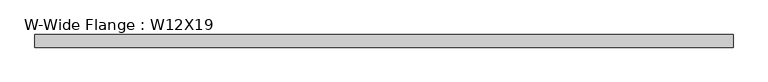
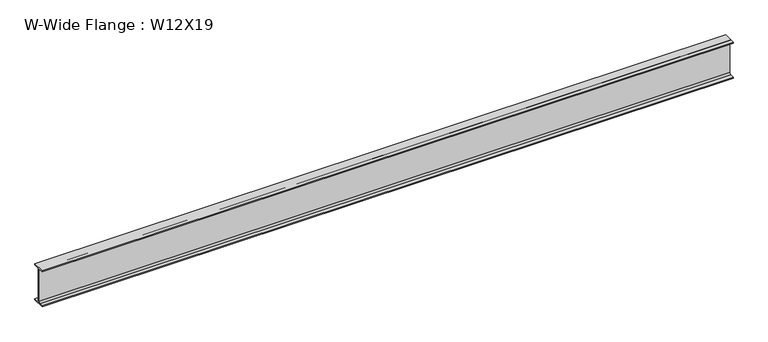
"""IFC4 building model written with IfcOpenShell, lengths in millimetres: beam geometry, W-Wide Flange : W12X19."""

from ifc_helpers import new_model, si_unit, point, frame, frame_2d, origin, place, context, project, spatial, polyline, circle_curve, trimmed, segment, composite_curve, outline, extrude, source, transform, mapped, element, save


def w_wide_flange_w12x19_30f12cce(model_context):
    return source(origin(), model_context, "Body", "SweptSolid", [
        extrude(outline(composite_curve([segment(polyline([(50.927, -146.05), (50.927, -154.94), (-50.927, -154.94), (-50.927, -146.05), (-16.3195, -146.05)]), True, "CONTINUOUS"), segment(trimmed(circle_curve(frame_2d((-16.3195, -132.715)), 13.335), [point((-16.3195, -146.05))], [point((-2.9845, -132.715))], True, "CARTESIAN"), True, "CONTINUOUS"), segment(polyline([(-2.9845, -132.715), (-2.9845, 132.715)]), True, "CONTINUOUS"), segment(trimmed(circle_curve(frame_2d((-16.3195, 132.715)), 13.335), [point((-2.9845, 132.715))], [point((-16.3195, 146.05))], True, "CARTESIAN"), True, "CONTINUOUS"), segment(polyline([(-16.3195, 146.05), (-50.927, 146.05), (-50.927, 154.94), (50.927, 154.94), (50.927, 146.05), (16.3195, 146.05)]), True, "CONTINUOUS"), segment(trimmed(circle_curve(frame_2d((16.3195, 132.715)), 13.335), [point((16.3195, 146.05))], [point((2.9845, 132.715))], True, "CARTESIAN"), True, "CONTINUOUS"), segment(polyline([(2.9845, 132.715), (2.9845, -132.715)]), True, "CONTINUOUS"), segment(trimmed(circle_curve(frame_2d((16.3195, -132.715)), 13.335), [point((2.9845, -132.715))], [point((16.3195, -146.05))], True, "CARTESIAN"), True, "CONTINUOUS"), segment(polyline([(16.3195, -146.05), (50.927, -146.05)]), True, "CONTINUOUS")], self_intersect=False)), frame((-2806.7, 0.0, 0.0), z_axis=(1.0, 0.0, 0.0), x_axis=(0.0, 1.0, 0.0)), (0.0, 0.0, 1.0), 5613.4),
    ])


if __name__ == "__main__":
    model = new_model("IFC4")
    model_context = context("Model", 3, world=origin())
    ifc_project = project(units=[si_unit("LENGTHUNIT", "METRE", prefix="MILLI")], contexts=[model_context])
    site = spatial("IfcSite", under=ifc_project)
    building = spatial("IfcBuilding", under=site)
    placement = place(None, origin())
    w_wide_flange_w12x19_shape = w_wide_flange_w12x19_30f12cce(model_context)
    element("IfcBeam", 1, ObjectType="W-Wide Flange : W12X19", at=placement, inside=building, context=model_context, shape_type="MappedRepresentation", body=[
        mapped(w_wide_flange_w12x19_shape, transform((0.0, 0.0, 0.0), x_axis=(1.0, 0.0, 0.0), y_axis=(0.0, 1.0, 0.0), z_axis=(0.0, 0.0, 1.0))),
    ])
    save(model, "model.ifc")

# Revit data of these elements
# Type "W-Wide Flange : W12X19"
#   Assembly Code = "B10"
#   W = 19
#   Length [instance default] = 5' - 0"
#   bf = 0' - 4.01"
#   d = 1' - 0.2"
#   k = 0' - 0 7/8"
#   k2 = 0' - 0.525"
#   tf = 0' - 0.35"
#   tw = 0' - 0.235"
#   A = 0.0386806 SF
#   Structural Material [instance default] = Steel ASTM A992
# Element 1 (IfcBeam, "W-Wide Flange : W12X19")
#   Materials on its faces: "Steel ASTM A992"
# Materials
#   "Steel ASTM A992": class "Metal", colour RGB 199 199 199, transparency 0, Description = "Structural steel 50ksi", Cost = 0
